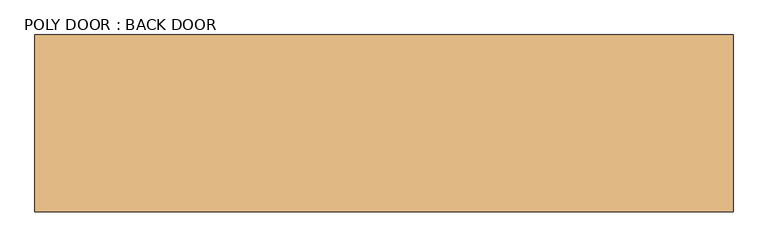
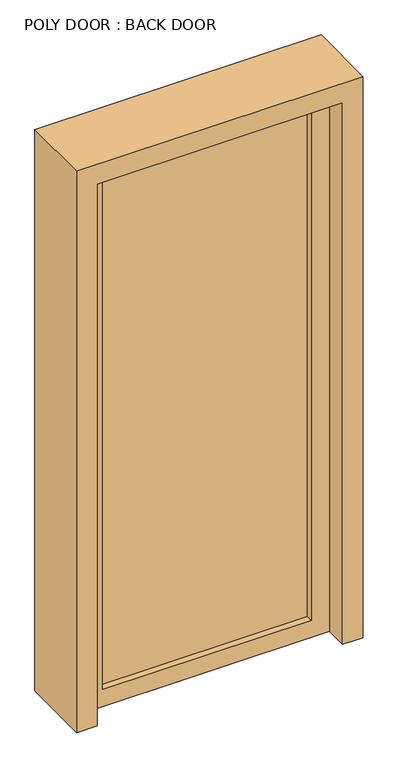
"""IFC4 building model written with IfcOpenShell, lengths in millimetres: door geometry, POLY DOOR : BACK DOOR."""

from ifc_helpers import new_model, si_unit, frame, origin, place, context, project, spatial, polyline, outline, extrude, source, transform, mapped, element, save


def poly_door_back_door_6149594f(model_context):
    return source(origin(), model_context, "Body", "SweptSolid", [
        extrude(outline(polyline([(388.9375, -25.4), (-388.9375, -25.4), (-388.9375, -12.7), (388.9375, -12.7), (388.9375, -25.4)])), frame((0.0, 0.0, 68.2625), z_axis=(0.0, 0.0, 1.0), x_axis=(1.0, 0.0, 0.0)), (0.0, 0.0, 1.0), 1997.075),
        extrude(outline(polyline([(2133.6, 457.2), (2133.6, -457.2), (0.0, -457.2), (0.0, 457.2), (2133.6, 457.2)]), holes=[polyline([(2065.3375, 388.9375), (68.2625, 388.9375), (68.2625, -388.9375), (2065.3375, -388.9375), (2065.3375, 388.9375)])]), frame((0.0, -50.8, 0.0), z_axis=(0.0, 1.0, 0.0), x_axis=(0.0, 0.0, 1.0)), (0.0, 0.0, 1.0), 50.8),
        extrude(outline(polyline([(2209.8, -533.4), (0.0, -533.4), (0.0, -457.2), (2133.6, -457.2), (2133.6, 457.2), (0.0, 457.2), (0.0, 533.4), (2209.8, 533.4), (2209.8, -533.4)])), frame((0.0, -134.9375, 0.0), z_axis=(0.0, 1.0, 0.0), x_axis=(0.0, 0.0, 1.0)), (0.0, 0.0, 1.0), 269.875),
    ])


if __name__ == "__main__":
    model = new_model("IFC4")
    model_context = context("Model", 3, world=origin())
    ifc_project = project(units=[si_unit("LENGTHUNIT", "METRE", prefix="MILLI")], contexts=[model_context])
    site = spatial("IfcSite", under=ifc_project)
    building = spatial("IfcBuilding", under=site)
    placement = place(None, origin())
    poly_door_back_door_shape = poly_door_back_door_6149594f(model_context)
    element("IfcDoor", 1, ObjectType="POLY DOOR : BACK DOOR", at=placement, inside=building, context=model_context, shape_type="MappedRepresentation", body=[
        mapped(poly_door_back_door_shape, transform((0.0, 0.0, 0.0), x_axis=(1.0, 0.0, 0.0), y_axis=(0.0, 1.0, 0.0), z_axis=(0.0, 0.0, 1.0))),
    ])
    save(model, "model.ifc")

# Revit data of these elements
# Type "POLY DOOR : BACK DOOR"
#   Type Mark = "64"
#   OD_DS_Door_Material = "ALUM./GLAZING"
#   OD_DS_Door_Type = "STOREFRONT (NARROW STILE)"
#   OD_DS_Lockset = "ENTRY LOCK (INSIDE ADA LEVER ALWAYS ACTIVE)"
#   Assembly Code = "C1020"
#   Analytic Construction = "<None>"
#   Thickness = 0' - 2"
#   Glass Inset = 0' - 2 11/16"
#   Height = 7' - 0"
#   Trim Projection Ext = 0' - 1"
#   Trim Projection Int = 0' - 1"
#   Trim Width = 0' - 3"
#   Width = 3' - 0"
#   WINDOW = yes
#   Glass Material = KAWNEER 260 INSULCLADTM THERMAL ENTRANCE - CLEAR ANODIZED ALUM.
#   Door Material = KAWNEER 260 INSULCLADTM THERMAL ENTRANCE - CLEAR ANODIZED ALUM.
#   Frame Material = KAWNEER TRIFAB VERSAGLAZE 451T - CLEAR ANODIZED ALUM. - BACK GLAZED
#   Function = (empty or 0)
#   Wall Closure = (empty or 0)
# Element 1 (IfcDoor, "POLY DOOR : BACK DOOR")
#   Materials on its faces: "KAWNEER 260 INSULCLADTM THERMAL ENTRANCE - CLEAR ANODIZED ALUM.", "KAWNEER TRIFAB VERSAGLAZE 451T - CLEAR ANODIZED ALUM. - BACK GLAZED"
# Materials
#   "KAWNEER 260 INSULCLADTM THERMAL ENTRANCE - CLEAR ANODIZED ALUM.": class "Metal", colour RGB 244 244 244, transparency 0, Description = "Aluminum 6061", Cost = 0
#   "KAWNEER TRIFAB VERSAGLAZE 451T - CLEAR ANODIZED ALUM. - BACK GLAZED": class "Metal", colour RGB 244 244 244, transparency 0, Description = "Aluminum 6061", Cost = 0
